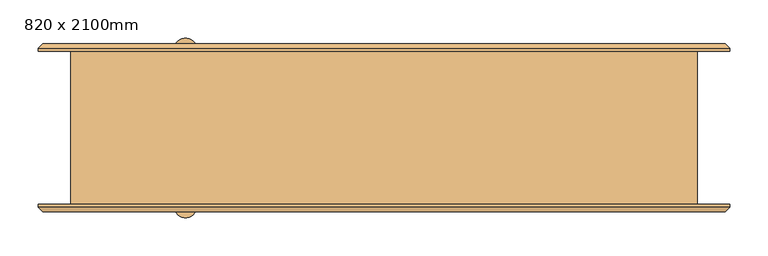
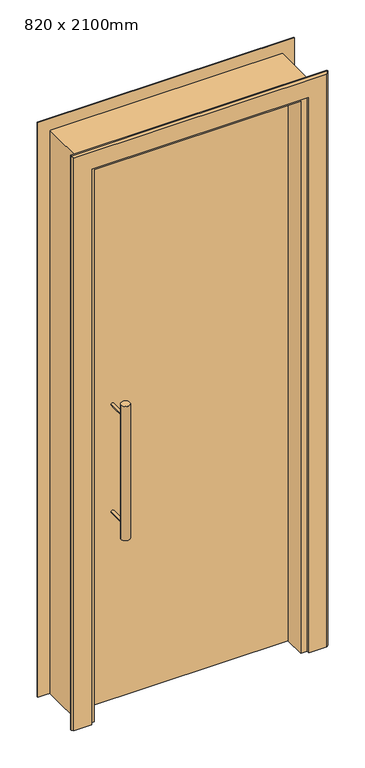
"""IFC4 building model written with IfcOpenShell, lengths in millimetres: door geometry, Porta pivotante simples com revestimento : 820 x 2100mm."""

from ifc_helpers import new_model, si_unit, point, frame, frame_2d, origin, origin_with_axes, place, context, project, spatial, polyline, circle_curve, trimmed, segment, composite_curve, outline, extrude, faceted_brep, source, transform, mapped, element, save


def door_820_x_2100mm_83ad22da(model_context):
    return source(origin(), model_context, "Body", "SolidModel", [
        extrude(outline(composite_curve([segment(trimmed(circle_curve(frame_2d((-260.0, 102.5)), 15.0), [point((-275.0, 102.5))], [point((-245.0, 102.5))], False, "CARTESIAN"), True, "CONTINUOUS"), segment(trimmed(circle_curve(frame_2d((-260.0, 102.5)), 15.0), [point((-245.0, 102.5))], [point((-275.0, 102.5))], False, "CARTESIAN"), True, "CONTINUOUS")], self_intersect=False)), frame((0.0, 0.0, 650.0), z_axis=(0.0, 0.0, 1.0), x_axis=(1.0, 0.0, 0.0)), (0.0, 0.0, 1.0), 500.0),
        extrude(outline(composite_curve([segment(trimmed(circle_curve(frame_2d((1100.0, -260.0)), 5.0), [point((1100.0, -265.0))], [point((1100.0, -255.0))], False, "CARTESIAN"), True, "CONTINUOUS"), segment(trimmed(circle_curve(frame_2d((1100.0, -260.0)), 5.0), [point((1100.0, -255.0))], [point((1100.0, -265.0))], False, "CARTESIAN"), True, "CONTINUOUS")], self_intersect=False)), frame((0.0, 22.5, 0.0), z_axis=(0.0, 1.0, 0.0), x_axis=(0.0, 0.0, 1.0)), (0.0, 0.0, 1.0), 80.0),
        extrude(outline(composite_curve([segment(trimmed(circle_curve(frame_2d((700.0, -260.0)), 5.0), [point((700.0, -265.0))], [point((700.0, -255.0))], False, "CARTESIAN"), True, "CONTINUOUS"), segment(trimmed(circle_curve(frame_2d((700.0, -260.0)), 5.0), [point((700.0, -255.0))], [point((700.0, -265.0))], False, "CARTESIAN"), True, "CONTINUOUS")], self_intersect=False)), frame((0.0, 22.5, 0.0), z_axis=(0.0, 1.0, 0.0), x_axis=(0.0, 0.0, 1.0)), (0.0, 0.0, 1.0), 80.0),
        extrude(outline(composite_curve([segment(trimmed(circle_curve(frame_2d((1100.0, -260.0)), 5.0), [point((1100.0, -265.0))], [point((1100.0, -255.0))], False, "CARTESIAN"), True, "CONTINUOUS"), segment(trimmed(circle_curve(frame_2d((1100.0, -260.0)), 5.0), [point((1100.0, -255.0))], [point((1100.0, -265.0))], False, "CARTESIAN"), True, "CONTINUOUS")], self_intersect=False)), frame((0.0, -102.5, 0.0), z_axis=(0.0, 1.0, 0.0), x_axis=(0.0, 0.0, 1.0)), (0.0, 0.0, 1.0), 80.0),
        extrude(outline(composite_curve([segment(trimmed(circle_curve(frame_2d((700.0, -260.0)), 5.0), [point((700.0, -265.0))], [point((700.0, -255.0))], False, "CARTESIAN"), True, "CONTINUOUS"), segment(trimmed(circle_curve(frame_2d((700.0, -260.0)), 5.0), [point((700.0, -255.0))], [point((700.0, -265.0))], False, "CARTESIAN"), True, "CONTINUOUS")], self_intersect=False)), frame((0.0, -102.5, 0.0), z_axis=(0.0, 1.0, 0.0), x_axis=(0.0, 0.0, 1.0)), (0.0, 0.0, 1.0), 80.0),
        extrude(outline(composite_curve([segment(trimmed(circle_curve(frame_2d((-260.0, -102.5)), 15.0), [point((-275.0, -102.5))], [point((-245.0, -102.5))], False, "CARTESIAN"), True, "CONTINUOUS"), segment(trimmed(circle_curve(frame_2d((-260.0, -102.5)), 15.0), [point((-245.0, -102.5))], [point((-275.0, -102.5))], False, "CARTESIAN"), True, "CONTINUOUS")], self_intersect=False)), frame((0.0, 0.0, 650.0), z_axis=(0.0, 0.0, 1.0), x_axis=(1.0, 0.0, 0.0)), (0.0, 0.0, 1.0), 500.0),
        extrude(outline(polyline([(370.0, 22.5), (370.0, -22.5), (-370.0, -22.5), (-370.0, 22.5), (370.0, 22.5)])), origin_with_axes(), (0.0, 0.0, 1.0), 2060.0),
        faceted_brep([(-453.0, 104.0, 0.0), (-447.0, 110.0, 0.0), (-383.0, 110.0, 0.0), (-383.0, 100.0, 0.0), (-453.0, 100.0, 0.0), (-453.0, 104.0, 2143.0), (-447.0, 110.0, 2137.0), (447.0, 110.0, 2137.0), (447.0, 110.0, 0.0), (383.0, 110.0, 0.0), (383.0, 110.0, 2073.0), (-383.0, 110.0, 2073.0), (-383.0, 100.0, 2073.0), (383.0, 100.0, 2073.0), (383.0, 100.0, 0.0), (453.0, 100.0, 0.0), (453.0, 100.0, 2143.0), (-453.0, 100.0, 2143.0), (453.0, 104.0, 2143.0), (453.0, 104.0, 0.0)], [[[0, 1, 2, 3, 4]], [[1, 0, 5, 6]], [[2, 1, 6, 7, 8, 9, 10, 11]], [[3, 2, 11, 12]], [[4, 3, 12, 13, 14, 15, 16, 17]], [[0, 4, 17, 5]], [[7, 18, 19, 8]], [[19, 15, 14, 9, 8]], [[13, 10, 9, 14]], [[18, 16, 15, 19]], [[6, 5, 18, 7]], [[12, 11, 10, 13]], [[5, 17, 16, 18]]]),
        faceted_brep([(453.0, -104.0, 0.0), (447.0, -110.0, 0.0), (383.0, -110.0, 0.0), (383.0, -100.0, 0.0), (453.0, -100.0, 0.0), (453.0, -104.0, 2143.0), (447.0, -110.0, 2137.0), (-447.0, -110.0, 2137.0), (-447.0, -110.0, 0.0), (-383.0, -110.0, 0.0), (-383.0, -110.0, 2073.0), (383.0, -110.0, 2073.0), (383.0, -100.0, 2073.0), (-383.0, -100.0, 2073.0), (-383.0, -100.0, 0.0), (-453.0, -100.0, 0.0), (-453.0, -100.0, 2143.0), (453.0, -100.0, 2143.0), (-453.0, -104.0, 2143.0), (-453.0, -104.0, 0.0)], [[[0, 1, 2, 3, 4]], [[1, 0, 5, 6]], [[2, 1, 6, 7, 8, 9, 10, 11]], [[3, 2, 11, 12]], [[4, 3, 12, 13, 14, 15, 16, 17]], [[0, 4, 17, 5]], [[7, 18, 19, 8]], [[19, 15, 14, 9, 8]], [[13, 10, 9, 14]], [[18, 16, 15, 19]], [[6, 5, 18, 7]], [[12, 11, 10, 13]], [[5, 17, 16, 18]]]),
        faceted_brep([(410.0, 100.0, 2100.0), (410.0, -100.0, 2100.0), (410.0, -100.0, 0.0), (410.0, 100.0, 0.0), (-410.0, -100.0, 2100.0), (-410.0, -100.0, 0.0), (-370.0, -100.0, 0.0), (-370.0, -100.0, 2060.0), (360.0, -100.0, 2060.0), (360.0, -100.0, 0.0), (370.0, 100.0, 0.0), (360.0, -22.5, 0.0), (370.0, -22.5, 0.0), (-410.0, 100.0, 0.0), (-410.0, 100.0, 2100.0), (370.0, 100.0, 2060.0), (-360.0, 100.0, 2060.0), (-360.0, 100.0, 0.0), (-360.0, 22.5, 0.0), (-370.0, 22.5, 0.0), (-370.0, 22.5, 2060.0), (360.0, -22.5, 2060.0), (370.0, -22.5, 2060.0), (-360.0, 22.5, 2060.0)], [[[0, 1, 2, 3]], [[4, 5, 6, 7, 8, 9, 2, 1]], [[10, 3, 2, 9, 11, 12]], [[13, 14, 0, 3, 10, 15, 16, 17]], [[4, 14, 13, 5]], [[13, 17, 18, 19, 6, 5]], [[6, 19, 20, 7]], [[11, 9, 8, 21]], [[10, 12, 22, 15]], [[18, 17, 16, 23]], [[12, 11, 21, 22]], [[19, 18, 23, 20]], [[21, 8, 7, 20, 23, 16, 15, 22]], [[1, 0, 14, 4]]]),
    ])


if __name__ == "__main__":
    model = new_model("IFC4")
    model_context = context("Model", 3, world=origin())
    ifc_project = project(units=[si_unit("LENGTHUNIT", "METRE", prefix="MILLI")], contexts=[model_context])
    site = spatial("IfcSite", under=ifc_project)
    building = spatial("IfcBuilding", under=site)
    placement = place(None, origin())
    door_820_x_2100mm_shape = door_820_x_2100mm_83ad22da(model_context)
    element("IfcDoor", 1, ObjectType="Porta pivotante simples com revestimento : 820 x 2100mm", at=placement, inside=building, context=model_context, shape_type="MappedRepresentation", body=[
        mapped(door_820_x_2100mm_shape, transform((0.0, 0.0, 0.0), x_axis=(1.0, 0.0, 0.0), y_axis=(0.0, 1.0, 0.0), z_axis=(0.0, 0.0, 1.0))),
    ])
    save(model, "model.ifc")

# Revit data of these elements
# Type "Porta pivotante simples com revestimento : 820 x 2100mm"
#   Type Mark = "35"
#   Construction Type Id = "MDOOR"
#   Analytic Construction = "Metal"
#   Largura da apara = 70 mm
#   Espessura da apara = 10 mm
#   Thickness = 45 mm
#   Rough Width = 820 mm
#   Rough Height = 2100 mm
#   Largura do painel = 740 mm
#   Sub-largura do painel = 120 mm
#   Heat Transfer Coefficient (U) = 3.7021 W/(m²·K)
#   Height = 2100 mm
#   Width = 820 mm
#   Largura da estrutura = 50 mm
#   Largura da moldura média = 40 mm
#   Function = 1
#   Material da apara = none
#   Material do painel = none
#   Material do puxador = none
#   Material da moldura = none
#   Visual Light Transmittance = 0
#   Solar Heat Gain Coefficient = 0
#   Wall Closure = (empty or 0)
